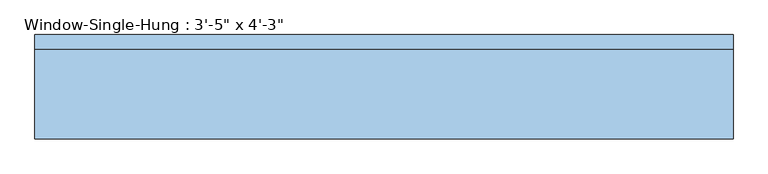
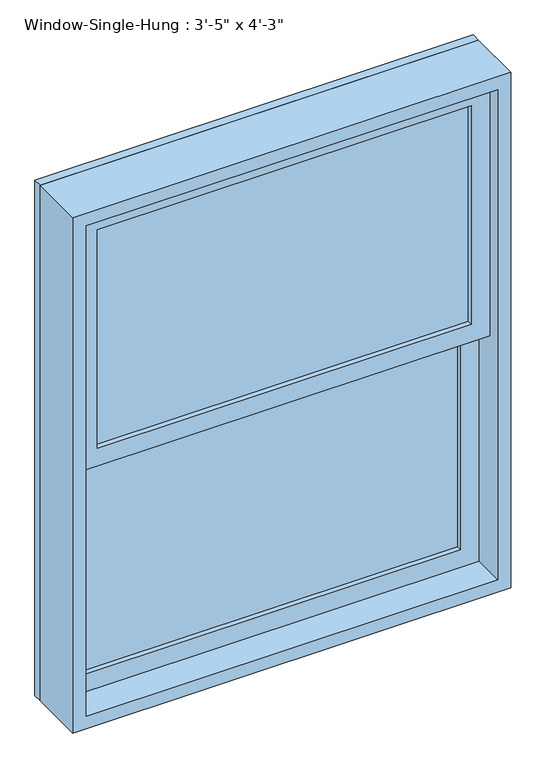
"""IFC4 building model written with IfcOpenShell, lengths in millimetres: window geometry."""

from ifc_helpers import new_model, si_unit, frame, origin, place, context, project, spatial, polyline, outline, extrude, source, transform, mapped, element, save


def window_8b75fed9(model_context):
    return source(origin(), model_context, "Body", "SweptSolid", [
        extrude(outline(polyline([(444.5, 1.5875), (-444.5, 1.5875), (-444.5, 7.9375), (444.5, 7.9375), (444.5, 1.5875)])), frame((0.0, 0.0, 990.6), z_axis=(0.0, 0.0, 1.0), x_axis=(1.0, 0.0, 0.0)), (0.0, 0.0, 1.0), 549.275),
        extrude(outline(polyline([(-444.5, 14.2875), (-444.5, 20.6375), (444.5, 20.6375), (444.5, 14.2875), (-444.5, 14.2875)])), frame((0.0, 0.0, 990.6), z_axis=(0.0, 0.0, 1.0), x_axis=(1.0, 0.0, 0.0)), (0.0, 0.0, 1.0), 549.275),
        extrude(outline(polyline([(444.5, -42.8625), (-444.5, -42.8625), (-444.5, -36.5125), (444.5, -36.5125), (444.5, -42.8625)])), frame((0.0, 0.0, 1584.325), z_axis=(0.0, 0.0, 1.0), x_axis=(1.0, 0.0, 0.0)), (0.0, 0.0, 1.0), 549.275),
        extrude(outline(polyline([(-444.5, -30.1625), (-444.5, -23.8125), (444.5, -23.8125), (444.5, -30.1625), (-444.5, -30.1625)])), frame((0.0, 0.0, 1584.325), z_axis=(0.0, 0.0, 1.0), x_axis=(1.0, 0.0, 0.0)), (0.0, 0.0, 1.0), 549.275),
        extrude(outline(polyline([(1584.325, 488.95), (1584.325, -488.95), (946.15, -488.95), (946.15, 488.95), (1584.325, 488.95)]), holes=[polyline([(1539.875, -444.5), (1539.875, 444.5), (990.6, 444.5), (990.6, -444.5), (1539.875, -444.5)])]), frame((0.0, -11.1125, 0.0), z_axis=(0.0, 1.0, 0.0), x_axis=(0.0, 0.0, 1.0)), (0.0, 0.0, 1.0), 44.45),
        extrude(outline(polyline([(2178.05, 488.95), (2178.05, -488.95), (1539.875, -488.95), (1539.875, 488.95), (2178.05, 488.95)]), holes=[polyline([(2133.6, -444.5), (2133.6, 444.5), (1584.325, 444.5), (1584.325, -444.5), (2133.6, -444.5)])]), frame((0.0, -55.5625, 0.0), z_axis=(0.0, 1.0, 0.0), x_axis=(0.0, 0.0, 1.0)), (0.0, 0.0, 1.0), 44.45),
        extrude(outline(polyline([(2209.8, 520.7), (2209.8, -520.7), (914.4, -520.7), (914.4, 520.7), (2209.8, 520.7)]), holes=[polyline([(2178.05, -488.95), (2178.05, 488.95), (946.15, 488.95), (946.15, -488.95), (2178.05, -488.95)])]), frame((0.0, -87.3125, 0.0), z_axis=(0.0, 1.0, 0.0), x_axis=(0.0, 0.0, 1.0)), (0.0, 0.0, 1.0), 133.35),
        extrude(outline(polyline([(2209.8, 520.7), (2209.8, -520.7), (914.4, -520.7), (914.4, 520.7), (2209.8, 520.7)]), holes=[polyline([(2190.75, 501.65), (933.45, 501.65), (933.45, -501.65), (2190.75, -501.65), (2190.75, 501.65)])]), frame((0.0, 46.0375, 0.0), z_axis=(0.0, 1.0, 0.0), x_axis=(0.0, 0.0, 1.0)), (0.0, 0.0, 1.0), 22.225),
    ])


if __name__ == "__main__":
    model = new_model("IFC4")
    model_context = context("Model", 3, world=origin())
    ifc_project = project(units=[si_unit("LENGTHUNIT", "METRE", prefix="MILLI")], contexts=[model_context])
    site = spatial("IfcSite", under=ifc_project)
    building = spatial("IfcBuilding", under=site)
    placement = place(None, origin())
    window_shape = window_8b75fed9(model_context)
    element("IfcWindow", 1, ObjectType="Window-Single-Hung : 3'-5\" x 4'-3\"", at=placement, inside=building, context=model_context, shape_type="MappedRepresentation", body=[
        mapped(window_shape, transform((0.0, 0.0, 0.0), x_axis=(1.0, 0.0, 0.0), y_axis=(0.0, 1.0, 0.0), z_axis=(0.0, 0.0, 1.0))),
    ])
    save(model, "model.ifc")

# Revit data of these elements
# Type "Window-Single-Hung : 3'-5\" x 4'-3\""
#   Type Mark = "26"
#   Fire Rating = "0.5h"
#   Construction Type Id = "DG-DR"
#   Assembly Code = "B2020100"
#   Analytic Construction = "Double glazing - domestic"
#   Wall Thickness [instance default] = 0' - 6"
#   Window Inset [instance default] = 0' - 0"
#   Visual Light Transmittance = 0.81
#   Thermal Resistance (R) = 0.319569 (m²·K)/W
#   Solar Heat Gain Coefficient = 0.76
#   Muntin Width = 2' - 11"
#   Muntin Height = 1' - 9 5/8"
#   Interior Wall Closure [instance default] = 0' - 1 1/2"
#   Rough Width = 3' - 5 1/2"
#   Rough Height = 4' - 3 1/2"
#   Frame Extension [instance default] = 0' - 1 1/4"
#   Exterior Wall Closure [instance default] = 0' - 0 1/2"
#   Extension Jamb [instance default] = 0' - 1 1/2"
#   Heat Transfer Coefficient (U) = 3.12929 W/(m²·K)
#   Height = 4' - 3"
#   Width = 3' - 5"
#   Top Muntin Visibility = yes
#   Indicator Visibility [instance default] = yes
#   Extension Jamb Visibility [instance default] = yes
#   Interior Trim Visibility [instance default] = yes
#   Exterior Trim Visibility [instance default] = yes
#   Bottom Muntin Visibility = yes
#   Muntin Pattern = Muntin Pattern_2x2 : Muntin Pattern_2x2
#   Interior Trim Material = Wood - Stained
#   Interior Trim = Trim-Window-Interior-Flat : Picture Frame
#   Exterior Trim Material = Clad - White
#   Exterior Trim = Trim-Window-Exterior-Flat : with Sill
#   Glass Panel Material = Glass
#   Exterior Frame Material = Clad - White
#   Interior Frame Material = Wood - Stained
#   Wall Closure = (empty or 0)
# Element 1 (IfcWindow, "Window-Single-Hung : 3'-5\" x 4'-3\"")
#   Wall Thickness = 0' - 5 3/8"
#   Extension Jamb = 0' - 0 7/8"
#   Materials on its faces: "Wood - Stained", "Glass", "Clad - White"
# Materials
#   "Wood - Stained": class "Wood", colour RGB 224 178 126, transparency 0, Cost = 0
#   "Clad - White": class "Wood", colour RGB 242 242 238, transparency 0, Cost = 0
#   "Glass": class "Glass", colour RGB 0 128 192, transparency 0.75, Description = "Soda Lime Glass", Cost = 0
